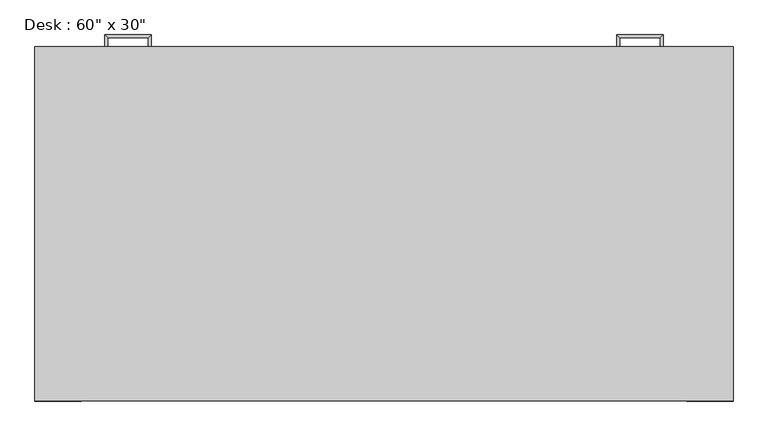
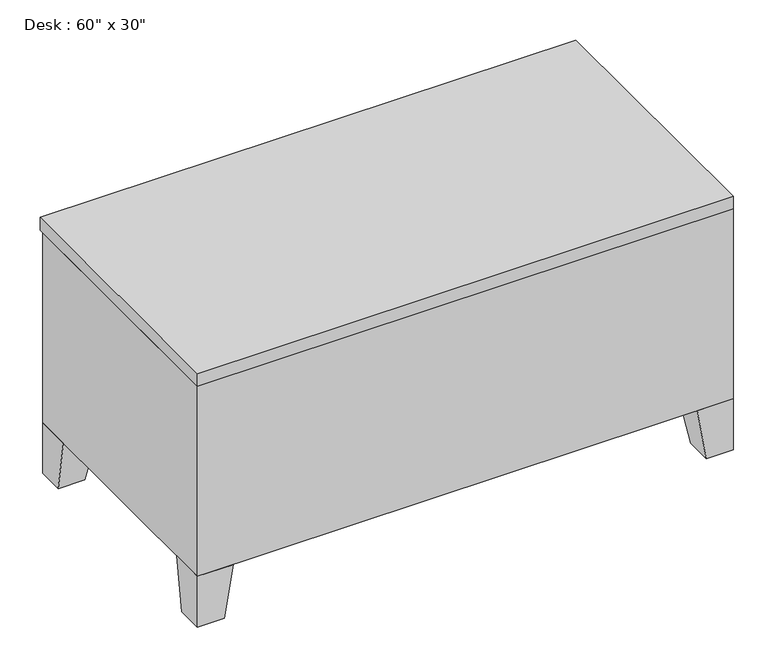
"""IFC4 building model written with IfcOpenShell, lengths in millimetres: furniture geometry."""

import ifcopenshell
import ifcopenshell.guid

model = None  # the IFC model being written
_history = None  # IfcOwnerHistory: only IFC2X3 demands one
_inside = {}  # id of a spatial element -> (the spatial element, [elements in it])
_under = {}  # id of a project, library or spatial element -> (it, [spatial elements below it])
_declared = {}  # id of a project -> (the project, [libraries it declares])
_typed = {}  # id of a type object -> (the type object, [elements of that type])
_made_of = {}  # id of a material, layer set ... -> (it, [elements and type objects made of it])


def new_model(schema):
    """Start an empty IFC model of exactly this schema.

    Asked for "IFC4X3", IfcOpenShell would pick the latest addendum, in which some entities
    have other attributes; the version numbers below select the first issue.
    IFC2X3 requires an IfcOwnerHistory on every rooted entity: one is made here for all.
    """
    global model, _history
    if schema == "IFC4X3":
        model = ifcopenshell.file(schema_version=(4, 3, 0, 0))
    else:
        model = ifcopenshell.file(schema=schema)
    _inside.clear()
    _under.clear()
    _declared.clear()
    _typed.clear()
    _made_of.clear()
    _history = None
    if model.schema == "IFC2X3":
        org = make("IfcOrganization", Name="unknown")
        user = make(
            "IfcPersonAndOrganization",
            ThePerson=make("IfcPerson", FamilyName="unknown"),
            TheOrganization=org,
        )
        app = make(
            "IfcApplication",
            ApplicationDeveloper=org,
            Version="unknown",
            ApplicationFullName="unknown",
            ApplicationIdentifier="unknown",
        )
        _history = make(
            "IfcOwnerHistory",
            OwningUser=user,
            OwningApplication=app,
            ChangeAction="ADDED",
            CreationDate=0,
        )
    return model


def make(cls, **values):
    """One entity of the class cls with the attributes given. An attribute that is None is left unset."""
    return model.create_entity(
        cls, **{name: value for name, value in values.items() if value is not None}
    )


def rooted(cls, **values):
    """An entity with a GlobalId (a new one), such as an element, a storey or a relation."""
    return make(cls, GlobalId=ifcopenshell.guid.new(), OwnerHistory=_history, **values)


def si_unit(unit_type, name, prefix=None):
    """IfcSIUnit, for example si_unit("LENGTHUNIT", "METRE", prefix="MILLI")."""
    return make("IfcSIUnit", UnitType=unit_type, Prefix=prefix, Name=name)


def assignment(units):
    """IfcUnitAssignment: the units of a project."""
    return None if units is None else make("IfcUnitAssignment", Units=units)


def point(xyz):
    """IfcCartesianPoint."""
    return None if xyz is None else make("IfcCartesianPoint", Coordinates=xyz)


def direction(xyz):
    """IfcDirection."""
    return None if xyz is None else make("IfcDirection", DirectionRatios=xyz)


def frame(location, z_axis=None, x_axis=None):
    """IfcAxis2Placement3D, a coordinate frame: its origin and axes. An axis left out is left unset."""
    return make(
        "IfcAxis2Placement3D",
        Location=point(location),
        Axis=direction(z_axis),
        RefDirection=direction(x_axis),
    )


def origin():
    """The frame at (0, 0, 0) with its axes left unset."""
    return frame((0.0, 0.0, 0.0))


def place(relative_to, where):
    """IfcLocalPlacement: puts the frame where relative to a parent placement (None: the world)."""
    return make(
        "IfcLocalPlacement", PlacementRelTo=relative_to, RelativePlacement=where
    )


def context(
    kind, dimensions, precision=None, world=None, true_north=None, identifier=None
):
    """IfcGeometricRepresentationContext, for example the 3D "Model" context."""
    return make(
        "IfcGeometricRepresentationContext",
        ContextIdentifier=identifier,
        ContextType=kind,
        CoordinateSpaceDimension=dimensions,
        Precision=precision,
        WorldCoordinateSystem=world,
        TrueNorth=true_north,
    )


def project(units=None, contexts=None):
    """IfcProject with its units and contexts."""
    return rooted(
        "IfcProject",
        Name="project",
        RepresentationContexts=contexts,
        UnitsInContext=assignment(units),
    )


def spatial(cls, under=None, at=None, **own):
    """A site, building, storey or space (cls), placed at a placement, below another one or the project."""
    s = rooted(cls, ObjectPlacement=at, **own)
    if under is not None:
        _under.setdefault(under.id(), (under, []))[1].append(s)
    return s


def polyline(points):
    """IfcPolyline through the points."""
    return make("IfcPolyline", Points=[point(p) for p in points])


def outline(outer, holes=None, kind="AREA"):
    """IfcArbitraryClosedProfileDef: a profile drawn as a closed curve; with holes, ...WithVoids."""
    if holes is None:
        return make("IfcArbitraryClosedProfileDef", ProfileType=kind, OuterCurve=outer)
    return make(
        "IfcArbitraryProfileDefWithVoids",
        ProfileType=kind,
        OuterCurve=outer,
        InnerCurves=holes,
    )


def extrude(swept, where, along, depth):
    """IfcExtrudedAreaSolid: the profile swept, set in the frame where, extruded along a direction by depth."""
    return make(
        "IfcExtrudedAreaSolid",
        SweptArea=swept,
        Position=where,
        ExtrudedDirection=direction(along),
        Depth=depth,
    )


def faces_of(points, faces, orient=None, outer=None):
    """IfcFace entities. A face is a list of loops; a loop is a list of indices into points, from 0.

    orient and outer hold one flag for each loop. By default every Orientation is true, the
    first loop of a face is its IfcFaceOuterBound and the others are IfcFaceBound.
    """
    made = []
    for i, loops in enumerate(faces):
        bounds = []
        for j, loop in enumerate(loops):
            is_outer = j == 0 if outer is None else outer[i][j]
            bounds.append(
                make(
                    "IfcFaceOuterBound" if is_outer else "IfcFaceBound",
                    Bound=make("IfcPolyLoop", Polygon=[points[k] for k in loop]),
                    Orientation=True if orient is None else orient[i][j],
                )
            )
        made.append(make("IfcFace", Bounds=bounds))
    return made


def faceted_brep(points, faces, orient=None, outer=None, voids=None):
    """IfcFacetedBrep: a solid bounded by flat faces; with voids (closed shells), ...WithVoids."""
    shared = [point(p) for p in points]
    hull = make("IfcClosedShell", CfsFaces=faces_of(shared, faces, orient, outer))
    if voids is None:
        return make("IfcFacetedBrep", Outer=hull)
    return make(
        "IfcFacetedBrepWithVoids",
        Outer=hull,
        Voids=[
            make(cls, CfsFaces=faces_of(shared, fs, o, b)) for cls, fs, o, b in voids
        ],
    )


def shape(context_of_items, identifier, shape_type, items):
    """IfcShapeRepresentation: the items that make up one representation, for example the "Body"."""
    return make(
        "IfcShapeRepresentation",
        ContextOfItems=context_of_items,
        RepresentationIdentifier=identifier,
        RepresentationType=shape_type,
        Items=items,
    )


def source(mapping_origin, context_of_items, identifier, shape_type, items):
    """IfcRepresentationMap: a shape defined once, which mapped items show again and again."""
    return make(
        "IfcRepresentationMap",
        MappingOrigin=mapping_origin,
        MappedRepresentation=shape(context_of_items, identifier, shape_type, items),
    )


def transform(
    local_origin,
    x_axis=None,
    y_axis=None,
    z_axis=None,
    scale=None,
    scale2=None,
    scale3=None,
    uniform=True,
):
    """IfcCartesianTransformationOperator3D, or its non-uniform kind. x_axis, y_axis, z_axis: its Axis1, 2, 3."""
    if uniform:
        return make(
            "IfcCartesianTransformationOperator3D",
            Axis1=direction(x_axis),
            Axis2=direction(y_axis),
            LocalOrigin=point(local_origin),
            Scale=scale,
            Axis3=direction(z_axis),
        )
    return make(
        "IfcCartesianTransformationOperator3DnonUniform",
        Axis1=direction(x_axis),
        Axis2=direction(y_axis),
        LocalOrigin=point(local_origin),
        Scale=scale,
        Axis3=direction(z_axis),
        Scale2=scale2,
        Scale3=scale3,
    )


def mapped(mapping_source, mapping_target):
    """IfcMappedItem: shows the shape of a source again, moved by a transform."""
    return make(
        "IfcMappedItem", MappingSource=mapping_source, MappingTarget=mapping_target
    )


def made_of(thing, what):
    """Note that an element or type object is made of a material, layer set ...; save() writes the relation."""
    if what is not None:
        _made_of.setdefault(what.id(), (what, []))[1].append(thing)
    return thing


def element(
    cls,
    number,
    at=None,
    inside=None,
    cuts=None,
    type_object=None,
    material=None,
    context=None,
    identifier="Body",
    shape_type=None,
    held_by="IfcProductDefinitionShape",
    body=None,
    shapes=None,
    **own,
):
    """One element of the class cls, such as IfcWall. Its Tag is "e" and its number.

    at: its placement. inside: the storey or other place that contains it. cuts: it is an
    opening in that element (IfcRelVoidsElement). A single representation is given by context,
    identifier, shape_type and body (its items); several are given by shapes. held_by: the class
    of the entity that holds the representations. save() writes the other relations.
    """
    e = rooted(cls, Tag="e%d" % number, ObjectPlacement=at, **own)
    if body is not None:
        shapes = [shape(context, identifier, shape_type, body)]
    if shapes is not None:
        e.Representation = make(held_by, Representations=shapes)
    if inside is not None:
        _inside.setdefault(inside.id(), (inside, []))[1].append(e)
    if cuts is not None:
        rooted(
            "IfcRelVoidsElement", RelatingBuildingElement=cuts, RelatedOpeningElement=e
        )
    if type_object is not None:
        _typed.setdefault(type_object.id(), (type_object, []))[1].append(e)
    return made_of(e, material)


def aggregate(whole, parts):
    """IfcRelAggregates: a whole, such as a stair, and the parts it consists of."""
    return rooted("IfcRelAggregates", RelatingObject=whole, RelatedObjects=parts)


def save(model, path):
    """Write the relations noted so far, then the file.

    IfcRelAggregates (storeys below a building ...), IfcRelContainedInSpatialStructure (elements
    in a storey), IfcRelDefinesByType, IfcRelAssociatesMaterial and IfcRelDeclares: one each for
    every whole, place, type object, material and project.
    """
    for whole, parts in _under.values():
        aggregate(whole, parts)
    for where, things in _inside.values():
        rooted(
            "IfcRelContainedInSpatialStructure",
            RelatedElements=things,
            RelatingStructure=where,
        )
    for kind, things in _typed.values():
        rooted("IfcRelDefinesByType", RelatedObjects=things, RelatingType=kind)
    for what, things in _made_of.values():
        rooted("IfcRelAssociatesMaterial", RelatedObjects=things, RelatingMaterial=what)
    for by, libraries in _declared.values():
        rooted("IfcRelDeclares", RelatingContext=by, RelatedDefinitions=libraries)
    model.write(path)


def furniture_e30ff25b(model_context):
    return source(origin(), model_context, "Body", "SolidModel", [
        extrude(outline(polyline([(19.05, 0.0), (19.05, 12.7), (387.35, 12.7), (387.35, 0.0), (19.05, 0.0)])), frame((0.0, 0.0, 603.25), z_axis=(0.0, 0.0, 1.0), x_axis=(1.0, 0.0, 0.0)), (0.0, 0.0, 1.0), 101.6),
        extrude(outline(polyline([(19.05, 0.0), (19.05, 12.7), (387.35, 12.7), (387.35, 0.0), (19.05, 0.0)])), frame((0.0, 0.0, 171.45), z_axis=(0.0, 0.0, 1.0), x_axis=(1.0, 0.0, 0.0)), (0.0, 0.0, 1.0), 412.75),
        extrude(outline(polyline([(1136.65, 0.0), (1136.65, 12.7), (1504.95, 12.7), (1504.95, 0.0), (1136.65, 0.0)])), frame((0.0, 0.0, 603.25), z_axis=(0.0, 0.0, 1.0), x_axis=(1.0, 0.0, 0.0)), (0.0, 0.0, 1.0), 101.6),
        extrude(outline(polyline([(1136.65, 0.0), (1136.65, 12.7), (1504.95, 12.7), (1504.95, 0.0), (1136.65, 0.0)])), frame((0.0, 0.0, 171.45), z_axis=(0.0, 0.0, 1.0), x_axis=(1.0, 0.0, 0.0)), (0.0, 0.0, 1.0), 171.45),
        extrude(outline(polyline([(1136.65, 0.0), (1136.65, 12.7), (1504.95, 12.7), (1504.95, 0.0), (1136.65, 0.0)])), frame((0.0, 0.0, 482.6), z_axis=(0.0, 0.0, 1.0), x_axis=(1.0, 0.0, 0.0)), (0.0, 0.0, 1.0), 101.6),
        extrude(outline(polyline([(1136.65, 0.0), (1136.65, 12.7), (1504.95, 12.7), (1504.95, 0.0), (1136.65, 0.0)])), frame((0.0, 0.0, 361.95), z_axis=(0.0, 0.0, 1.0), x_axis=(1.0, 0.0, 0.0)), (0.0, 0.0, 1.0), 101.6),
        faceted_brep([(101.6, 0.0, 152.4), (0.0, 0.0, 152.4), (0.0, -101.6, 152.4), (101.6, -101.6, 152.4), (76.2, 0.0, 0.0), (76.2, -76.2, 0.0), (0.0, -76.2, 0.0), (0.0, 0.0, 0.0)], [[[0, 1, 2, 3]], [[4, 5, 6, 7]], [[4, 0, 3, 5]], [[5, 3, 2, 6]], [[6, 2, 1, 7]], [[7, 1, 0, 4]]]),
        faceted_brep([(101.6, -762.0, 152.4), (101.6, -660.4, 152.4), (0.0, -660.4, 152.4), (0.0, -762.0, 152.4), (76.2, -762.0, 0.0), (0.0, -762.0, 0.0), (0.0, -685.8, 0.0), (76.2, -685.8, 0.0)], [[[0, 1, 2, 3]], [[4, 5, 6, 7]], [[4, 0, 3, 5]], [[5, 3, 2, 6]], [[6, 2, 1, 7]], [[7, 1, 0, 4]]]),
        faceted_brep([(1422.4, -762.0, 152.4), (1524.0, -762.0, 152.4), (1524.0, -660.4, 152.4), (1422.4, -660.4, 152.4), (1447.8, -762.0, 0.0), (1447.8, -685.8, 0.0), (1524.0, -685.8, 0.0), (1524.0, -762.0, 0.0)], [[[0, 1, 2, 3]], [[4, 5, 6, 7]], [[4, 0, 3, 5]], [[5, 3, 2, 6]], [[6, 2, 1, 7]], [[7, 1, 0, 4]]]),
        faceted_brep([(1422.4, 0.0, 152.4), (1422.4, -101.6, 152.4), (1524.0, -101.6, 152.4), (1524.0, 0.0, 152.4), (1447.8, 0.0, 0.0), (1524.0, 0.0, 0.0), (1524.0, -76.2, 0.0), (1447.8, -76.2, 0.0)], [[[0, 1, 2, 3]], [[4, 5, 6, 7]], [[4, 0, 3, 5]], [[5, 3, 2, 6]], [[6, 2, 1, 7]], [[7, 1, 0, 4]]]),
        extrude(outline(polyline([(0.0, 12.7), (1524.0, 12.7), (1524.0, -762.0), (0.0, -762.0), (0.0, 12.7)])), frame((0.0, 0.0, 723.9), z_axis=(0.0, 0.0, 1.0), x_axis=(1.0, 0.0, 0.0)), (0.0, 0.0, 1.0), 38.1),
        extrude(outline(polyline([(1117.6, 0.0), (1524.0, 0.0), (1524.0, -762.0), (0.0, -762.0), (0.0, 0.0), (406.4, 0.0), (406.4, -635.0), (1117.6, -635.0), (1117.6, 0.0)])), frame((0.0, 0.0, 152.4), z_axis=(0.0, 0.0, 1.0), x_axis=(1.0, 0.0, 0.0)), (0.0, 0.0, 1.0), 571.5),
        faceted_brep([(158.75, 12.7, 546.1), (152.4, 12.7, 546.1), (152.4, 12.7, 533.4), (158.75, 12.7, 533.4), (158.75, 31.75, 533.4), (158.75, 31.75, 546.1), (152.4, 38.1, 533.4), (152.4, 38.1, 546.1), (247.65, 31.75, 533.4), (247.65, 31.75, 546.1), (254.0, 38.1, 533.4), (254.0, 38.1, 546.1), (247.65, 12.7, 546.1), (247.65, 12.7, 533.4), (254.0, 12.7, 533.4), (254.0, 12.7, 546.1)], [[[0, 1, 2, 3]], [[3, 4, 5, 0]], [[2, 6, 4, 3]], [[1, 7, 6, 2]], [[0, 5, 7, 1]], [[4, 8, 9, 5]], [[6, 10, 8, 4]], [[7, 11, 10, 6]], [[5, 9, 11, 7]], [[12, 13, 14, 15]], [[8, 13, 12, 9]], [[10, 14, 13, 8]], [[11, 15, 14, 10]], [[9, 12, 15, 11]]]),
        faceted_brep([(158.75, 12.7, 666.75), (152.4, 12.7, 666.75), (152.4, 12.7, 654.05), (158.75, 12.7, 654.05), (158.75, 31.75, 654.05), (158.75, 31.75, 666.75), (152.4, 38.1, 654.05), (152.4, 38.1, 666.75), (247.65, 31.75, 654.05), (247.65, 31.75, 666.75), (254.0, 38.1, 654.05), (254.0, 38.1, 666.75), (247.65, 12.7, 666.75), (247.65, 12.7, 654.05), (254.0, 12.7, 654.05), (254.0, 12.7, 666.75)], [[[0, 1, 2, 3]], [[3, 4, 5, 0]], [[2, 6, 4, 3]], [[1, 7, 6, 2]], [[0, 5, 7, 1]], [[4, 8, 9, 5]], [[6, 10, 8, 4]], [[7, 11, 10, 6]], [[5, 9, 11, 7]], [[12, 13, 14, 15]], [[8, 13, 12, 9]], [[10, 14, 13, 8]], [[11, 15, 14, 10]], [[9, 12, 15, 11]]]),
        faceted_brep([(1365.25, 12.7, 304.8), (1365.25, 12.7, 292.1), (1371.6, 12.7, 292.1), (1371.6, 12.7, 304.8), (1371.6, 38.1, 304.8), (1365.25, 31.75, 304.8), (1371.6, 38.1, 292.1), (1365.25, 31.75, 292.1), (1270.0, 38.1, 304.8), (1276.35, 31.75, 304.8), (1270.0, 38.1, 292.1), (1276.35, 31.75, 292.1), (1276.35, 12.7, 304.8), (1270.0, 12.7, 304.8), (1270.0, 12.7, 292.1), (1276.35, 12.7, 292.1)], [[[0, 1, 2, 3]], [[3, 4, 5, 0]], [[2, 6, 4, 3]], [[1, 7, 6, 2]], [[0, 5, 7, 1]], [[4, 8, 9, 5]], [[6, 10, 8, 4]], [[7, 11, 10, 6]], [[5, 9, 11, 7]], [[12, 13, 14, 15]], [[8, 13, 12, 9]], [[10, 14, 13, 8]], [[11, 15, 14, 10]], [[9, 12, 15, 11]]]),
        faceted_brep([(1365.25, 12.7, 425.45), (1365.25, 12.7, 412.75), (1371.6, 12.7, 412.75), (1371.6, 12.7, 425.45), (1371.6, 38.1, 425.45), (1365.25, 31.75, 425.45), (1371.6, 38.1, 412.75), (1365.25, 31.75, 412.75), (1270.0, 38.1, 425.45), (1276.35, 31.75, 425.45), (1270.0, 38.1, 412.75), (1276.35, 31.75, 412.75), (1276.35, 12.7, 425.45), (1270.0, 12.7, 425.45), (1270.0, 12.7, 412.75), (1276.35, 12.7, 412.75)], [[[0, 1, 2, 3]], [[3, 4, 5, 0]], [[2, 6, 4, 3]], [[1, 7, 6, 2]], [[0, 5, 7, 1]], [[4, 8, 9, 5]], [[6, 10, 8, 4]], [[7, 11, 10, 6]], [[5, 9, 11, 7]], [[12, 13, 14, 15]], [[8, 13, 12, 9]], [[10, 14, 13, 8]], [[11, 15, 14, 10]], [[9, 12, 15, 11]]]),
        faceted_brep([(1365.25, 12.7, 546.1), (1365.25, 12.7, 533.4), (1371.6, 12.7, 533.4), (1371.6, 12.7, 546.1), (1371.6, 38.1, 546.1), (1365.25, 31.75, 546.1), (1371.6, 38.1, 533.4), (1365.25, 31.75, 533.4), (1270.0, 38.1, 546.1), (1276.35, 31.75, 546.1), (1270.0, 38.1, 533.4), (1276.35, 31.75, 533.4), (1276.35, 12.7, 546.1), (1270.0, 12.7, 546.1), (1270.0, 12.7, 533.4), (1276.35, 12.7, 533.4)], [[[0, 1, 2, 3]], [[3, 4, 5, 0]], [[2, 6, 4, 3]], [[1, 7, 6, 2]], [[0, 5, 7, 1]], [[4, 8, 9, 5]], [[6, 10, 8, 4]], [[7, 11, 10, 6]], [[5, 9, 11, 7]], [[12, 13, 14, 15]], [[8, 13, 12, 9]], [[10, 14, 13, 8]], [[11, 15, 14, 10]], [[9, 12, 15, 11]]]),
        faceted_brep([(1365.25, 12.7, 666.75), (1365.25, 12.7, 654.05), (1371.6, 12.7, 654.05), (1371.6, 12.7, 666.75), (1371.6, 38.1, 666.75), (1365.25, 31.75, 666.75), (1371.6, 38.1, 654.05), (1365.25, 31.75, 654.05), (1270.0, 38.1, 666.75), (1276.35, 31.75, 666.75), (1270.0, 38.1, 654.05), (1276.35, 31.75, 654.05), (1276.35, 12.7, 666.75), (1270.0, 12.7, 666.75), (1270.0, 12.7, 654.05), (1276.35, 12.7, 654.05)], [[[0, 1, 2, 3]], [[3, 4, 5, 0]], [[2, 6, 4, 3]], [[1, 7, 6, 2]], [[0, 5, 7, 1]], [[4, 8, 9, 5]], [[6, 10, 8, 4]], [[7, 11, 10, 6]], [[5, 9, 11, 7]], [[12, 13, 14, 15]], [[8, 13, 12, 9]], [[10, 14, 13, 8]], [[11, 15, 14, 10]], [[9, 12, 15, 11]]]),
    ])


if __name__ == "__main__":
    model = new_model("IFC4")
    model_context = context("Model", 3, world=origin())
    ifc_project = project(units=[si_unit("LENGTHUNIT", "METRE", prefix="MILLI")], contexts=[model_context])
    site = spatial("IfcSite", under=ifc_project)
    building = spatial("IfcBuilding", under=site)
    placement = place(None, origin())
    furniture_shape = furniture_e30ff25b(model_context)
    element("IfcFurniture", 1, ObjectType="Desk : 60\" x 30\"", at=placement, inside=building, context=model_context, shape_type="MappedRepresentation", body=[
        mapped(furniture_shape, transform((0.0, 0.0, 0.0), x_axis=(1.0, 0.0, 0.0), y_axis=(0.0, 1.0, 0.0), z_axis=(0.0, 0.0, 1.0))),
    ])
    save(model, "model.ifc")

# Revit data of these elements
# Type "Desk : 60\" x 30\""
#   Assembly Code = "E2020200"
#   Depth = 2' - 6"
#   Height = 2' - 6"
#   Leg Height = 0' - 6"
#   Width = 5' - 0"
#   Body Material = Laminate, Ivory, Matte
#   Handle/Leg Material = Steel, Chrome Plated
#   Top Material = Cherry
#   Default Elevation = 0
# Element 1 (IfcFurniture, "Desk : 60\" x 30\"")
#   Materials on its faces: "Steel, Chrome Plated", "Laminate, Ivory, Matte", "Cherry"
# Materials
#   "Laminate, Ivory, Matte": class "Plastic", colour RGB 247 247 239, transparency 0, Description = "Plastic Laminate - Ivory, Matte", Cost = 0
#   "Steel, Chrome Plated": class "Metal", colour RGB 17 17 17, transparency 0, Description = "Chromiuim plated steel", Cost = 0
#   "Cherry": class "Wood", colour RGB 226 177 128, transparency 0, Description = "Prunus Serotina", Cost = 0
